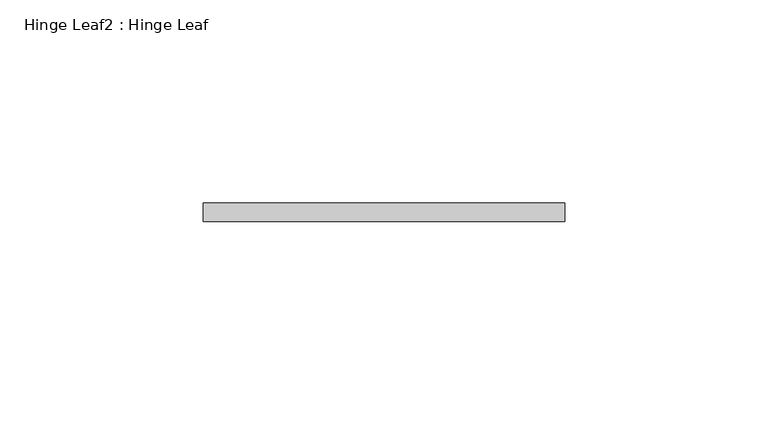
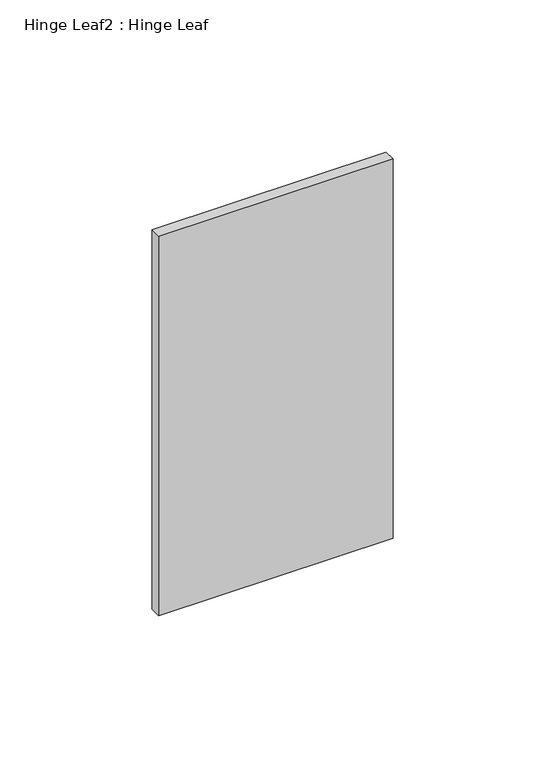
"""IFC4 building model written with IfcOpenShell, lengths in millimetres: proxy geometry, Hinge Leaf2 : Hinge Leaf."""

from ifc_helpers import new_model, si_unit, frame, origin, place, context, project, spatial, polyline, outline, extrude, source, transform, mapped, element, save


def hinge_leaf2_hinge_leaf_155bf624(model_context):
    return source(origin(), model_context, "Body", "SweptSolid", [
        extrude(outline(polyline([(587327.7934739, -531780.6943841), (587416.6934739, -531780.6943841), (587416.6934739, -531785.2663841), (587327.7934739, -531785.2663841), (587327.7934739, -531780.6943841)])), frame((0.0, 0.0, 311.15), z_axis=(0.0, 0.0, 1.0), x_axis=(1.0, 0.0, 0.0)), (0.0, 0.0, 1.0), 152.4),
    ])


if __name__ == "__main__":
    model = new_model("IFC4")
    model_context = context("Model", 3, world=origin())
    ifc_project = project(units=[si_unit("LENGTHUNIT", "METRE", prefix="MILLI")], contexts=[model_context])
    site = spatial("IfcSite", under=ifc_project)
    building = spatial("IfcBuilding", under=site)
    placement = place(None, origin())
    hinge_leaf2_hinge_leaf_shape = hinge_leaf2_hinge_leaf_155bf624(model_context)
    element("IfcBuildingElementProxy", 1, Name="Hinge Leaf2 : Hinge Leaf", ObjectType="Hinge Leaf2 : Hinge Leaf", at=placement, inside=building, context=model_context, shape_type="MappedRepresentation", body=[
        mapped(hinge_leaf2_hinge_leaf_shape, transform((0.0, 0.0, 0.0), x_axis=(1.0, 0.0, 0.0), y_axis=(0.0, 1.0, 0.0), z_axis=(0.0, 0.0, 1.0))),
    ])
    save(model, "model.ifc")

# Revit data of these elements
# Element 1 (IfcBuildingElementProxy, "Hinge Leaf2 : Hinge Leaf")
#   Materials on its faces: "6\"X6\" WELD-ON STL BUTT HINGE"
# Materials
#   "6\"X6\" WELD-ON STL BUTT HINGE": class "Metal", colour RGB 189 187 185, transparency 0, Description = "Carbon steel", Cost = 0
